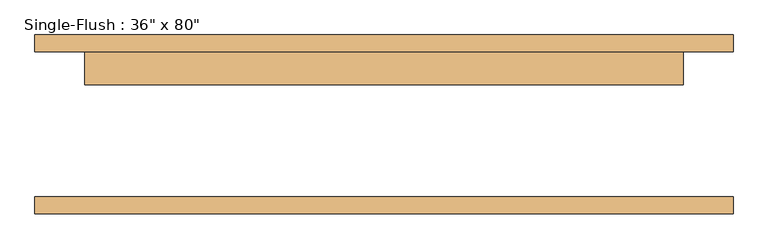
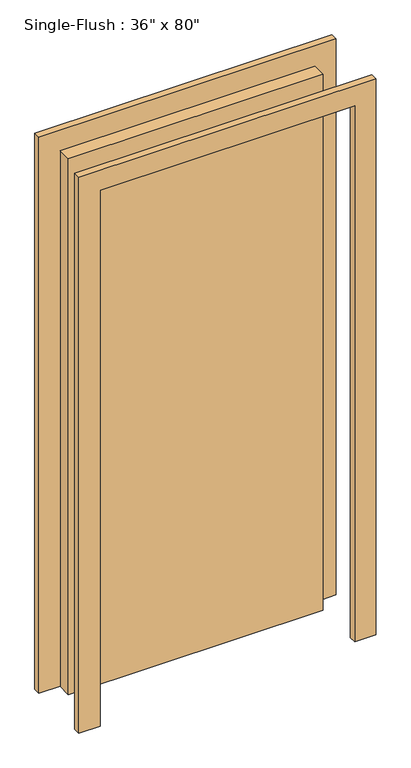
"""IFC4 building model written with IfcOpenShell, lengths in millimetres: door geometry."""

import ifcopenshell
import ifcopenshell.guid

model = None  # the IFC model being written
_history = None  # IfcOwnerHistory: only IFC2X3 demands one
_inside = {}  # id of a spatial element -> (the spatial element, [elements in it])
_under = {}  # id of a project, library or spatial element -> (it, [spatial elements below it])
_declared = {}  # id of a project -> (the project, [libraries it declares])
_typed = {}  # id of a type object -> (the type object, [elements of that type])
_made_of = {}  # id of a material, layer set ... -> (it, [elements and type objects made of it])


def new_model(schema):
    """Start an empty IFC model of exactly this schema.

    Asked for "IFC4X3", IfcOpenShell would pick the latest addendum, in which some entities
    have other attributes; the version numbers below select the first issue.
    IFC2X3 requires an IfcOwnerHistory on every rooted entity: one is made here for all.
    """
    global model, _history
    if schema == "IFC4X3":
        model = ifcopenshell.file(schema_version=(4, 3, 0, 0))
    else:
        model = ifcopenshell.file(schema=schema)
    _inside.clear()
    _under.clear()
    _declared.clear()
    _typed.clear()
    _made_of.clear()
    _history = None
    if model.schema == "IFC2X3":
        org = make("IfcOrganization", Name="unknown")
        user = make(
            "IfcPersonAndOrganization",
            ThePerson=make("IfcPerson", FamilyName="unknown"),
            TheOrganization=org,
        )
        app = make(
            "IfcApplication",
            ApplicationDeveloper=org,
            Version="unknown",
            ApplicationFullName="unknown",
            ApplicationIdentifier="unknown",
        )
        _history = make(
            "IfcOwnerHistory",
            OwningUser=user,
            OwningApplication=app,
            ChangeAction="ADDED",
            CreationDate=0,
        )
    return model


def make(cls, **values):
    """One entity of the class cls with the attributes given. An attribute that is None is left unset."""
    return model.create_entity(
        cls, **{name: value for name, value in values.items() if value is not None}
    )


def rooted(cls, **values):
    """An entity with a GlobalId (a new one), such as an element, a storey or a relation."""
    return make(cls, GlobalId=ifcopenshell.guid.new(), OwnerHistory=_history, **values)


def si_unit(unit_type, name, prefix=None):
    """IfcSIUnit, for example si_unit("LENGTHUNIT", "METRE", prefix="MILLI")."""
    return make("IfcSIUnit", UnitType=unit_type, Prefix=prefix, Name=name)


def assignment(units):
    """IfcUnitAssignment: the units of a project."""
    return None if units is None else make("IfcUnitAssignment", Units=units)


def point(xyz):
    """IfcCartesianPoint."""
    return None if xyz is None else make("IfcCartesianPoint", Coordinates=xyz)


def direction(xyz):
    """IfcDirection."""
    return None if xyz is None else make("IfcDirection", DirectionRatios=xyz)


def frame(location, z_axis=None, x_axis=None):
    """IfcAxis2Placement3D, a coordinate frame: its origin and axes. An axis left out is left unset."""
    return make(
        "IfcAxis2Placement3D",
        Location=point(location),
        Axis=direction(z_axis),
        RefDirection=direction(x_axis),
    )


def origin():
    """The frame at (0, 0, 0) with its axes left unset."""
    return frame((0.0, 0.0, 0.0))


def origin_with_axes():
    """The frame at (0, 0, 0) with the z axis (0, 0, 1) and the x axis (1, 0, 0) written out."""
    return frame((0.0, 0.0, 0.0), z_axis=(0.0, 0.0, 1.0), x_axis=(1.0, 0.0, 0.0))


def place(relative_to, where):
    """IfcLocalPlacement: puts the frame where relative to a parent placement (None: the world)."""
    return make(
        "IfcLocalPlacement", PlacementRelTo=relative_to, RelativePlacement=where
    )


def context(
    kind, dimensions, precision=None, world=None, true_north=None, identifier=None
):
    """IfcGeometricRepresentationContext, for example the 3D "Model" context."""
    return make(
        "IfcGeometricRepresentationContext",
        ContextIdentifier=identifier,
        ContextType=kind,
        CoordinateSpaceDimension=dimensions,
        Precision=precision,
        WorldCoordinateSystem=world,
        TrueNorth=true_north,
    )


def project(units=None, contexts=None):
    """IfcProject with its units and contexts."""
    return rooted(
        "IfcProject",
        Name="project",
        RepresentationContexts=contexts,
        UnitsInContext=assignment(units),
    )


def spatial(cls, under=None, at=None, **own):
    """A site, building, storey or space (cls), placed at a placement, below another one or the project."""
    s = rooted(cls, ObjectPlacement=at, **own)
    if under is not None:
        _under.setdefault(under.id(), (under, []))[1].append(s)
    return s


def polyline(points):
    """IfcPolyline through the points."""
    return make("IfcPolyline", Points=[point(p) for p in points])


def outline(outer, holes=None, kind="AREA"):
    """IfcArbitraryClosedProfileDef: a profile drawn as a closed curve; with holes, ...WithVoids."""
    if holes is None:
        return make("IfcArbitraryClosedProfileDef", ProfileType=kind, OuterCurve=outer)
    return make(
        "IfcArbitraryProfileDefWithVoids",
        ProfileType=kind,
        OuterCurve=outer,
        InnerCurves=holes,
    )


def extrude(swept, where, along, depth):
    """IfcExtrudedAreaSolid: the profile swept, set in the frame where, extruded along a direction by depth."""
    return make(
        "IfcExtrudedAreaSolid",
        SweptArea=swept,
        Position=where,
        ExtrudedDirection=direction(along),
        Depth=depth,
    )


def shape(context_of_items, identifier, shape_type, items):
    """IfcShapeRepresentation: the items that make up one representation, for example the "Body"."""
    return make(
        "IfcShapeRepresentation",
        ContextOfItems=context_of_items,
        RepresentationIdentifier=identifier,
        RepresentationType=shape_type,
        Items=items,
    )


def source(mapping_origin, context_of_items, identifier, shape_type, items):
    """IfcRepresentationMap: a shape defined once, which mapped items show again and again."""
    return make(
        "IfcRepresentationMap",
        MappingOrigin=mapping_origin,
        MappedRepresentation=shape(context_of_items, identifier, shape_type, items),
    )


def transform(
    local_origin,
    x_axis=None,
    y_axis=None,
    z_axis=None,
    scale=None,
    scale2=None,
    scale3=None,
    uniform=True,
):
    """IfcCartesianTransformationOperator3D, or its non-uniform kind. x_axis, y_axis, z_axis: its Axis1, 2, 3."""
    if uniform:
        return make(
            "IfcCartesianTransformationOperator3D",
            Axis1=direction(x_axis),
            Axis2=direction(y_axis),
            LocalOrigin=point(local_origin),
            Scale=scale,
            Axis3=direction(z_axis),
        )
    return make(
        "IfcCartesianTransformationOperator3DnonUniform",
        Axis1=direction(x_axis),
        Axis2=direction(y_axis),
        LocalOrigin=point(local_origin),
        Scale=scale,
        Axis3=direction(z_axis),
        Scale2=scale2,
        Scale3=scale3,
    )


def mapped(mapping_source, mapping_target):
    """IfcMappedItem: shows the shape of a source again, moved by a transform."""
    return make(
        "IfcMappedItem", MappingSource=mapping_source, MappingTarget=mapping_target
    )


def made_of(thing, what):
    """Note that an element or type object is made of a material, layer set ...; save() writes the relation."""
    if what is not None:
        _made_of.setdefault(what.id(), (what, []))[1].append(thing)
    return thing


def element(
    cls,
    number,
    at=None,
    inside=None,
    cuts=None,
    type_object=None,
    material=None,
    context=None,
    identifier="Body",
    shape_type=None,
    held_by="IfcProductDefinitionShape",
    body=None,
    shapes=None,
    **own,
):
    """One element of the class cls, such as IfcWall. Its Tag is "e" and its number.

    at: its placement. inside: the storey or other place that contains it. cuts: it is an
    opening in that element (IfcRelVoidsElement). A single representation is given by context,
    identifier, shape_type and body (its items); several are given by shapes. held_by: the class
    of the entity that holds the representations. save() writes the other relations.
    """
    e = rooted(cls, Tag="e%d" % number, ObjectPlacement=at, **own)
    if body is not None:
        shapes = [shape(context, identifier, shape_type, body)]
    if shapes is not None:
        e.Representation = make(held_by, Representations=shapes)
    if inside is not None:
        _inside.setdefault(inside.id(), (inside, []))[1].append(e)
    if cuts is not None:
        rooted(
            "IfcRelVoidsElement", RelatingBuildingElement=cuts, RelatedOpeningElement=e
        )
    if type_object is not None:
        _typed.setdefault(type_object.id(), (type_object, []))[1].append(e)
    return made_of(e, material)


def aggregate(whole, parts):
    """IfcRelAggregates: a whole, such as a stair, and the parts it consists of."""
    return rooted("IfcRelAggregates", RelatingObject=whole, RelatedObjects=parts)


def save(model, path):
    """Write the relations noted so far, then the file.

    IfcRelAggregates (storeys below a building ...), IfcRelContainedInSpatialStructure (elements
    in a storey), IfcRelDefinesByType, IfcRelAssociatesMaterial and IfcRelDeclares: one each for
    every whole, place, type object, material and project.
    """
    for whole, parts in _under.values():
        aggregate(whole, parts)
    for where, things in _inside.values():
        rooted(
            "IfcRelContainedInSpatialStructure",
            RelatedElements=things,
            RelatingStructure=where,
        )
    for kind, things in _typed.values():
        rooted("IfcRelDefinesByType", RelatedObjects=things, RelatingType=kind)
    for what, things in _made_of.values():
        rooted("IfcRelAssociatesMaterial", RelatedObjects=things, RelatingMaterial=what)
    for by, libraries in _declared.values():
        rooted("IfcRelDeclares", RelatingContext=by, RelatedDefinitions=libraries)
    model.write(path)


def door_521908aa(model_context):
    return source(origin(), model_context, "Body", "SweptSolid", [
        extrude(outline(polyline([(2108.2, -533.4), (0.0, -533.4), (0.0, -457.2), (2032.0, -457.2), (2032.0, 457.2), (0.0, 457.2), (0.0, 533.4), (2108.2, 533.4), (2108.2, -533.4)])), frame((0.0, 111.125, 0.0), z_axis=(0.0, 1.0, 0.0), x_axis=(0.0, 0.0, 1.0)), (0.0, 0.0, 1.0), 25.4),
        extrude(outline(polyline([(2108.2, 533.4), (2108.2, -533.4), (0.0, -533.4), (0.0, -457.2), (2032.0, -457.2), (2032.0, 457.2), (0.0, 457.2), (0.0, 533.4), (2108.2, 533.4)])), frame((0.0, -136.525, 0.0), z_axis=(0.0, 1.0, 0.0), x_axis=(0.0, 0.0, 1.0)), (0.0, 0.0, 1.0), 25.4),
        extrude(outline(polyline([(457.2, 60.325), (-457.2, 60.325), (-457.2, 111.125), (457.2, 111.125), (457.2, 60.325)])), origin_with_axes(), (0.0, 0.0, 1.0), 2032.0),
    ])


if __name__ == "__main__":
    model = new_model("IFC4")
    model_context = context("Model", 3, world=origin())
    ifc_project = project(units=[si_unit("LENGTHUNIT", "METRE", prefix="MILLI")], contexts=[model_context])
    site = spatial("IfcSite", under=ifc_project)
    building = spatial("IfcBuilding", under=site)
    placement = place(None, origin())
    door_shape = door_521908aa(model_context)
    element("IfcDoor", 1, ObjectType="Single-Flush : 36\" x 80\"", at=placement, inside=building, context=model_context, shape_type="MappedRepresentation", body=[
        mapped(door_shape, transform((0.0, 0.0, 0.0), x_axis=(1.0, 0.0, 0.0), y_axis=(0.0, 1.0, 0.0), z_axis=(0.0, 0.0, 1.0))),
    ])
    save(model, "model.ifc")

# Revit data of these elements
# Type "Single-Flush : 36\" x 80\""
#   Type Mark = "13"
#   Construction Type Id = "MDOOR"
#   Assembly Code = "C1020"
#   Analytic Construction = "Metal"
#   Thickness = 0' - 2"
#   Heat Transfer Coefficient (U) = 3.7021 W/(m²·K)
#   Height = 6' - 8"
#   Trim Projection Ext = 0' - 1"
#   Trim Projection Int = 0' - 1"
#   Trim Width = 0' - 3"
#   Width = 3' - 0"
#   Door Material = Aluminum
#   Frame Material = Aluminum
#   Visual Light Transmittance = 0
#   Solar Heat Gain Coefficient = 0
#   Function = (empty or 0)
#   Wall Closure = (empty or 0)
# Element 1 (IfcDoor, "Single-Flush : 36\" x 80\"")
#   Materials on its faces: "Aluminum"
# Materials
#   "Aluminum": class "Metal", colour RGB 226 226 226, transparency 0, Description = "Aluminum 6061", Cost = 0
